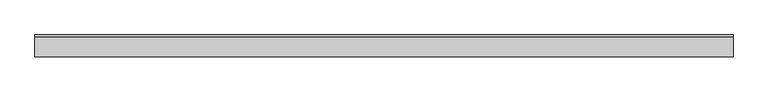
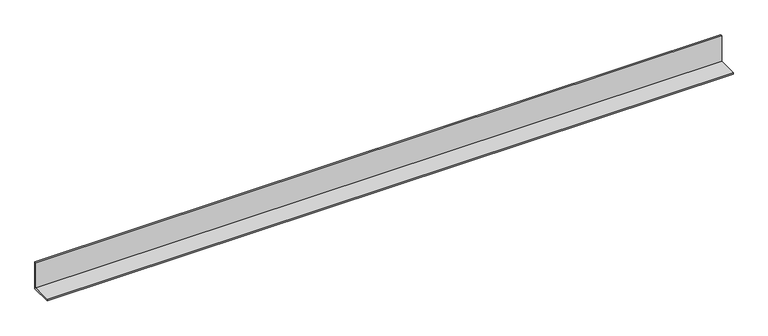
"""IFC4 building model written with IfcOpenShell, lengths in millimetres: proxy geometry, Generic Models 3:Generic Models 1:6:Generic Models 1:6 : Generic Models 3:Generic Models 1:300625:350611:Generic Models 1:6:Generic Models 1:6 : Generic Models 3:Generic Models 1:300625:350611 : Generic Models 3:Generic Models 1:6:Generic Models 1:6 : Generic Models 3:Generic Models 1:300625:350611:1 : Generic Models 3:Generic Models 1:6:Generic Models 1:6 : Generic Models 3:Generic Models 1:300625:350611:Generic Models 1:6:Generic Models 1:6 : Generic Models 3:Generic Models 1:300625:350611 : Generic Models 3:Generic Models 1:6:Generic Models 1:6 : Generic Models 3:Generic Models 1:300625:350611:301824."""

from ifc_helpers import new_model, si_unit, frame, origin, place, context, project, spatial, polyline, outline, extrude, source, transform, mapped, element, save


def generic_models_aaa7de9f(model_context):
    return source(origin(), model_context, "Body", "SweptSolid", [
        extrude(outline(polyline([(-578797.4913841, 0.0), (-578873.6913841, 0.0), (-578873.6913841, 6.35), (-578803.8413841, 6.35), (-578803.8413841, 101.6), (-578797.4913841, 101.6), (-578797.4913841, 0.0)])), frame((593738.0867239, 0.0, 0.0), z_axis=(1.0, 0.0, 0.0), x_axis=(0.0, 1.0, 0.0)), (0.0, 0.0, 1.0), 2438.4),
    ])


if __name__ == "__main__":
    model = new_model("IFC4")
    model_context = context("Model", 3, world=origin())
    ifc_project = project(units=[si_unit("LENGTHUNIT", "METRE", prefix="MILLI")], contexts=[model_context])
    site = spatial("IfcSite", under=ifc_project)
    building = spatial("IfcBuilding", under=site)
    placement = place(None, origin())
    generic_models_shape = generic_models_aaa7de9f(model_context)
    element("IfcBuildingElementProxy", 1, Name="Generic Models 3:Generic Models 1:6:Generic Models 1:6 : Generic Models 3:Generic Models 1:300625:350611:Generic Models 1:6:Generic Models 1:6 : Generic Models 3:Generic Models 1:300625:350611 : Generic Models 3:Generic Models 1:6:Generic Models 1:6 : Generic Models 3:Generic Models 1:300625:350611:1 : Generic Models 3:Generic Models 1:6:Generic Models 1:6 : Generic Models 3:Generic Models 1:300625:350611:Generic Models 1:6:Generic Models 1:6 : Generic Models 3:Generic Models 1:300625:350611 : Generic Models 3:Generic Models 1:6:Generic Models 1:6 : Generic Models 3:Generic Models 1:300625:350611:301824", ObjectType="Generic Models 3:Generic Models 1:6:Generic Models 1:6 : Generic Models 3:Generic Models 1:300625:350611:Generic Models 1:6:Generic Models 1:6 : Generic Models 3:Generic Models 1:300625:350611 : Generic Models 3:Generic Models 1:6:Generic Models 1:6 : Generic Models 3:Generic Models 1:300625:350611:1 : Generic Models 3:Generic Models 1:6:Generic Models 1:6 : Generic Models 3:Generic Models 1:300625:350611:Generic Models 1:6:Generic Models 1:6 : Generic Models 3:Generic Models 1:300625:350611 : Generic Models 3:Generic Models 1:6:Generic Models 1:6 : Generic Models 3:Generic Models 1:300625:350611:301824", at=placement, inside=building, context=model_context, shape_type="MappedRepresentation", body=[
        mapped(generic_models_shape, transform((0.0, 0.0, 0.0), x_axis=(1.0, 0.0, 0.0), y_axis=(0.0, 1.0, 0.0), z_axis=(0.0, 0.0, 1.0))),
    ])
    save(model, "model.ifc")

# Revit data of these elements
# Type "Generic Models 3:Generic Models 1:6:Generic Models 1:6 : Generic Models 3:Generic Models 1:300625:350611:Generic Models 1:6:Generic Models 1:6 : Generic Models 3:Generic Models 1:300625:350611 : Generic Models 3:Generic Models 1:6:Generic Models 1:6 : Generic Models 3:Generic Models 1:300625:350611:1 : Generic Models 3:Generic Models 1:6:Generic Models 1:6 : Generic Models 3:Generic Models 1:300625:350611:Generic Models 1:6:Generic Models 1:6 : Generic Models 3:Generic Models 1:300625:350611 : Generic Models 3:Generic Models 1:6:Generic Models 1:6 : Generic Models 3:Generic Models 1:300625:350611:301824"
#   NameOverride = "Generic Models 3:Generic Models 1:6:Generic Models 1:6 : Generic Models 3:Generic Models 1:300625:350611:Generic Models 1:6:Generic Models 1:6 : Generic Models 3:Generic Models 1:300625:350611 : Generic Models 3:Generic Models 1:6:Generic Models 1:6 : Generic Models 3:Generic Models 1:300625:350611:301824"
#   ObjectTypeOverride = "Generic Models 1:6:Generic Models 1:6 : Generic Models 3:Generic Models 1:300625:350611 : Generic Models 3:Generic Models 1:6:Generic Models 1:6 : Generic Models 3:Generic Models 1:300625:350611"
#   Reference = "Generic Models 1"
#   Tag = "301824"
# Element 1 (IfcBuildingElementProxy, "Generic Models 3:Generic Models 1:6:Generic Models 1:6 : Generic Models 3:Generic Models 1:300625:350611:Generic Models 1:6:Generic Models 1:6 : Generic Models 3:Generic Models 1:300625:350611 : Generic Models 3:Generic Models 1:6:Generic Models 1:6 : Generic Models 3:Generic Models 1:300625:350611:1 : Generic Models 3:Generic Models 1:6:Generic Models 1:6 : Generic Models 3:Generic Models 1:300625:350611:Generic Models 1:6:Generic Models 1:6 : Generic Models 3:Generic Models 1:300625:350611 : Generic Models 3:Generic Models 1:6:Generic Models 1:6 : Generic Models 3:Generic Models 1:300625:350611:301824")
#   Materials on its faces: "6\" Metal Stud Track_1"
# Materials
#   "6\" Metal Stud Track_1": class "Unassigned", colour RGB 120 120 120, transparency 0
